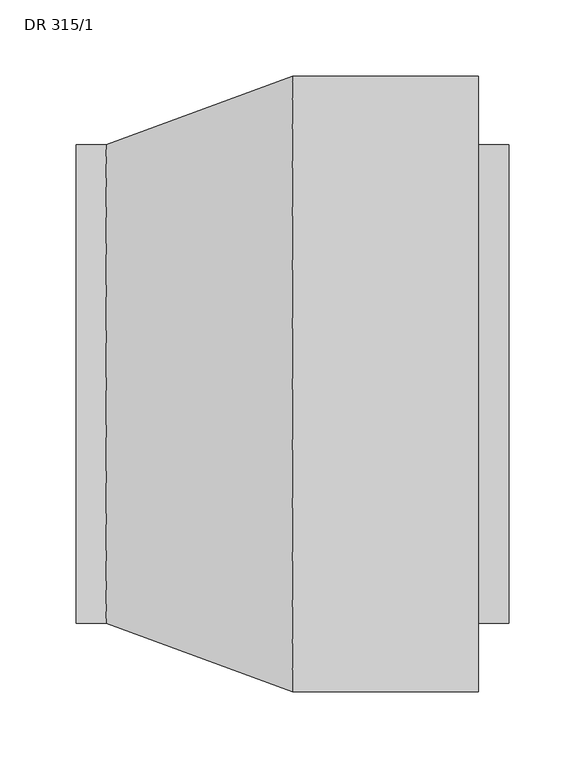
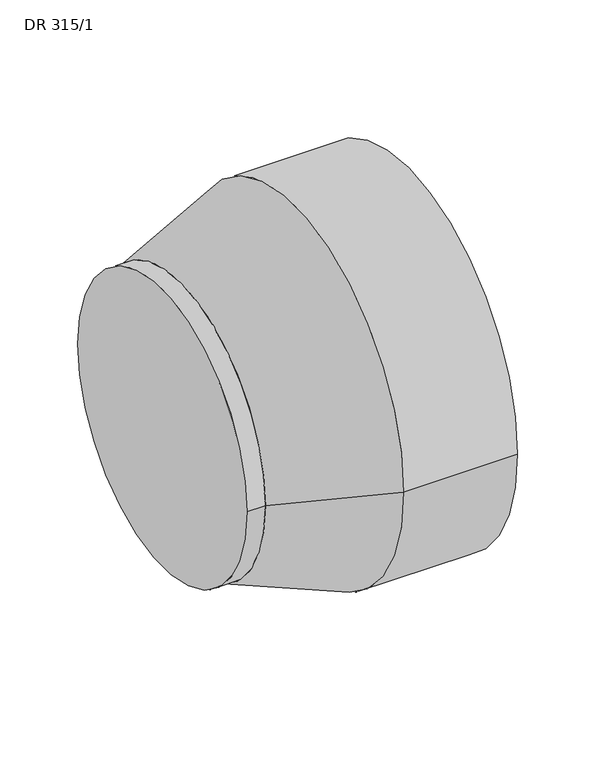
"""IFC4 building model written with IfcOpenShell, lengths in millimetres: proxy geometry, Канальный вентилятор DR : DR 315/1."""

from ifc_helpers import new_model, si_unit, point, frame, origin, origin_2d, place, context, project, spatial, polyline, circle_curve, trimmed, segment, composite_curve, outline, extrude, source, transform, mapped, element, save
from ifc_brep_helpers import plane_surface, revolved_surface, advanced_brep


def dr_315_1_fd02a15b(model_context):
    return source(origin(), model_context, "Body", "SolidModel", [
        advanced_brep(
        [(-122.5, -157.5, 0.0), (-122.5, 157.5, 0.0), (0.0, -202.5, 0.0), (0.0, 202.5, 0.0)],
        [
            (0, 1, circle_curve(frame((-122.5, 0.0, 0.0), z_axis=(-1.0, 0.0, 0.0), x_axis=(0.0, -1.0, 0.0)), 157.5)),
            (1, 0, circle_curve(frame((-122.5, 0.0, 0.0), z_axis=(-1.0, 0.0, 0.0), x_axis=(0.0, 1.0, 0.0)), 157.5)),
            (2, 3, circle_curve(frame((0.0, 0.0, 0.0), z_axis=(1.0, 0.0, 0.0), x_axis=(0.0, 1.0, 0.0)), 202.5)),
            (3, 2, circle_curve(frame((0.0, 0.0, 0.0), z_axis=(1.0, 0.0, 0.0), x_axis=(0.0, -1.0, 0.0)), 202.5)),
            (2, 0),
            (1, 3),
        ],
        [
            plane_surface(frame((-122.5, 0.0, 0.0), z_axis=(-1.0, 0.0, 0.0), x_axis=(0.0, 0.0, -1.0))),
            plane_surface(frame((0.0, 0.0, 0.0), z_axis=(1.0, 0.0, 0.0), x_axis=(0.0, 0.0, -1.0))),
            revolved_surface(polyline([(-122.5, 157.5, 0.0), (0.0, 202.5, 0.0)]), (-551.25, 0.0, 0.0), (1.0, 0.0, 0.0)),
            revolved_surface(polyline([(-122.5, -157.5, 0.0), (0.0, -202.5, 0.0)]), (-551.25, 0.0, 0.0), (1.0, 0.0, 0.0)),
        ],
        [
            (0, [[1, 2]]),
            (1, [[3, 4]]),
            (2, [[-3, 5, -2, 6]]),
            (3, [[-4, -6, -1, -5]]),
        ],
    ),
        extrude(outline(composite_curve([segment(trimmed(circle_curve(origin_2d(), 157.5), [point((-157.5, 0.0))], [point((157.5, 0.0))], False, "CARTESIAN"), True, "CONTINUOUS"), segment(trimmed(circle_curve(origin_2d(), 157.5), [point((157.5, 0.0))], [point((-157.5, 0.0))], False, "CARTESIAN"), True, "CONTINUOUS")], self_intersect=False)), frame((-142.5, 0.0, 0.0), z_axis=(1.0, 0.0, 0.0), x_axis=(0.0, 1.0, 0.0)), (0.0, 0.0, 1.0), 20.0),
        extrude(outline(composite_curve([segment(trimmed(circle_curve(origin_2d(), 202.5), [point((-202.5, 0.0))], [point((202.5, 0.0))], False, "CARTESIAN"), True, "CONTINUOUS"), segment(trimmed(circle_curve(origin_2d(), 202.5), [point((202.5, 0.0))], [point((-202.5, 0.0))], False, "CARTESIAN"), True, "CONTINUOUS")], self_intersect=False)), frame((0.0, 0.0, 0.0), z_axis=(1.0, 0.0, 0.0), x_axis=(0.0, 1.0, 0.0)), (0.0, 0.0, 1.0), 122.5),
        extrude(outline(composite_curve([segment(trimmed(circle_curve(origin_2d(), 157.5), [point((-157.5, 0.0))], [point((157.5, 0.0))], False, "CARTESIAN"), True, "CONTINUOUS"), segment(trimmed(circle_curve(origin_2d(), 157.5), [point((157.5, 0.0))], [point((-157.5, 0.0))], False, "CARTESIAN"), True, "CONTINUOUS")], self_intersect=False)), frame((122.5, 0.0, 0.0), z_axis=(1.0, 0.0, 0.0), x_axis=(0.0, 1.0, 0.0)), (0.0, 0.0, 1.0), 20.0),
    ])


if __name__ == "__main__":
    model = new_model("IFC4")
    model_context = context("Model", 3, world=origin())
    ifc_project = project(units=[si_unit("LENGTHUNIT", "METRE", prefix="MILLI")], contexts=[model_context])
    site = spatial("IfcSite", under=ifc_project)
    building = spatial("IfcBuilding", under=site)
    placement = place(None, origin())
    dr_315_1_shape = dr_315_1_fd02a15b(model_context)
    element("IfcBuildingElementProxy", 1, Name="Канальный вентилятор DR : DR 315/1", ObjectType="Канальный вентилятор DR : DR 315/1", at=placement, inside=building, context=model_context, shape_type="MappedRepresentation", body=[
        mapped(dr_315_1_shape, transform((0.0, 0.0, 0.0), x_axis=(1.0, 0.0, 0.0), y_axis=(0.0, 1.0, 0.0), z_axis=(0.0, 0.0, 1.0))),
    ])
    save(model, "model.ifc")

# Revit data of these elements
# Type "Канальный вентилятор DR : DR 315/1"
#   Manufacturer = "WAER"
#   ADSK_Система_Имя [instance default] = ""
#   ADSK_Наименование краткое = "DR 315/1"
#   ADSK_Наименование [instance default] = "Канальный вентилятор DR 315/1"
#   ADSK_Масса_Текст = "6"
#   ADSK_Марка = ""
#   ADSK_Код изделия = ""
#   ADSK_Завод-изготовитель = "WAER"
#   ADSK_Единица измерения = "шт."
#   ADSK_URL страницы изделия = ""
#   ADSK_URL документации изделия = ""
#   ADSK_Ток = 1.2 A
#   ADSK_Расход воздуха = 0 m³/h
#   ADSK_Размер_Длина_В = 285 mm
#   ADSK_Размер_Диаметр_С = 405 mm
#   ADSK_Размер_Диаметр_А = 315 mm
#   ADSK_Потеря давления воздуха = 180.0 Pa
#   ADSK_Полная мощность = 1.2 VA
#   ADSK_Номинальная мощность = 270 W
#   ADSK_Напряжение = 1 V
#   ADSK_Масса = 6
#   ADSK_Количество [instance default] = 1
#   ADSK_Количество фаз = 1
#   ADSK_Классификация нагрузок = ОВК
#   Default Elevation = 0
#   URL = ""
#   Cost = 0
